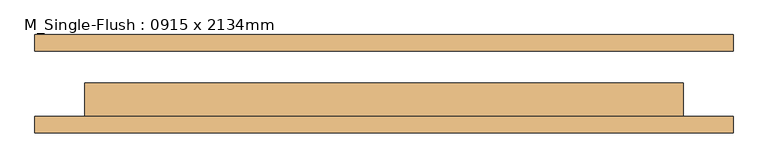
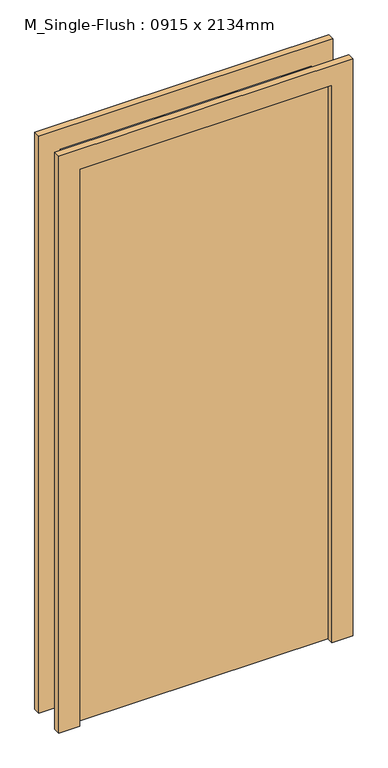
"""IFC4 building model written with IfcOpenShell, lengths in millimetres: door geometry, M_Single-Flush : 0915 x 2134mm."""

from ifc_helpers import new_model, si_unit, frame, origin, origin_with_axes, place, context, project, spatial, polyline, outline, extrude, source, transform, mapped, element, save


def m_single_flush_0915_x_2134mm_17617764(model_context):
    return source(origin(), model_context, "Body", "SweptSolid", [
        extrude(outline(polyline([(2210.0, -533.5), (0.0, -533.5), (0.0, -457.5), (2134.0, -457.5), (2134.0, 457.5), (0.0, 457.5), (0.0, 533.5), (2210.0, 533.5), (2210.0, -533.5)])), frame((0.0, -75.0, 0.0), z_axis=(0.0, 1.0, 0.0), x_axis=(0.0, 0.0, 1.0)), (0.0, 0.0, 1.0), 25.0),
        extrude(outline(polyline([(2210.0, 533.5), (2210.0, -533.5), (0.0, -533.5), (0.0, -457.5), (2134.0, -457.5), (2134.0, 457.5), (0.0, 457.5), (0.0, 533.5), (2210.0, 533.5)])), frame((0.0, 50.0, 0.0), z_axis=(0.0, 1.0, 0.0), x_axis=(0.0, 0.0, 1.0)), (0.0, 0.0, 1.0), 25.0),
        extrude(outline(polyline([(457.5, 1.0), (457.5, -50.0), (-457.5, -50.0), (-457.5, 1.0), (457.5, 1.0)])), origin_with_axes(), (0.0, 0.0, 1.0), 2134.0),
    ])


if __name__ == "__main__":
    model = new_model("IFC4")
    model_context = context("Model", 3, world=origin())
    ifc_project = project(units=[si_unit("LENGTHUNIT", "METRE", prefix="MILLI")], contexts=[model_context])
    site = spatial("IfcSite", under=ifc_project)
    building = spatial("IfcBuilding", under=site)
    placement = place(None, origin())
    m_single_flush_0915_x_2134mm_shape = m_single_flush_0915_x_2134mm_17617764(model_context)
    element("IfcDoor", 1, ObjectType="M_Single-Flush : 0915 x 2134mm", at=placement, inside=building, context=model_context, shape_type="MappedRepresentation", body=[
        mapped(m_single_flush_0915_x_2134mm_shape, transform((0.0, 0.0, 0.0), x_axis=(1.0, 0.0, 0.0), y_axis=(0.0, 1.0, 0.0), z_axis=(0.0, 0.0, 1.0))),
    ])
    save(model, "model.ifc")

# Revit data of these elements
# Type "M_Single-Flush : 0915 x 2134mm"
#   Type Mark = "15"
#   Thickness = 5.1 cm
#   Height = 213.4 cm
#   Trim Projection Ext = 2.5 cm
#   Trim Projection Int = 2.5 cm
#   Trim Width = 7.6 cm
#   Width = 91.5 cm
#   Door Material = Door - Panel
#   Frame Material = Door - Frame
#   Function = (empty or 0)
#   Wall Closure = (empty or 0)
# Element 1 (IfcDoor, "M_Single-Flush : 0915 x 2134mm")
#   Materials on its faces: "Door - Frame", "Door - Panel"
# Materials
#   "Door - Panel": class "Wood", colour RGB 114 82 51, transparency 0
#   "Door - Frame": class "Miscellaneous", colour RGB 153 76 43, transparency 0
